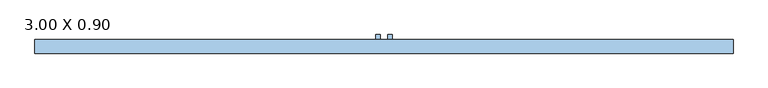
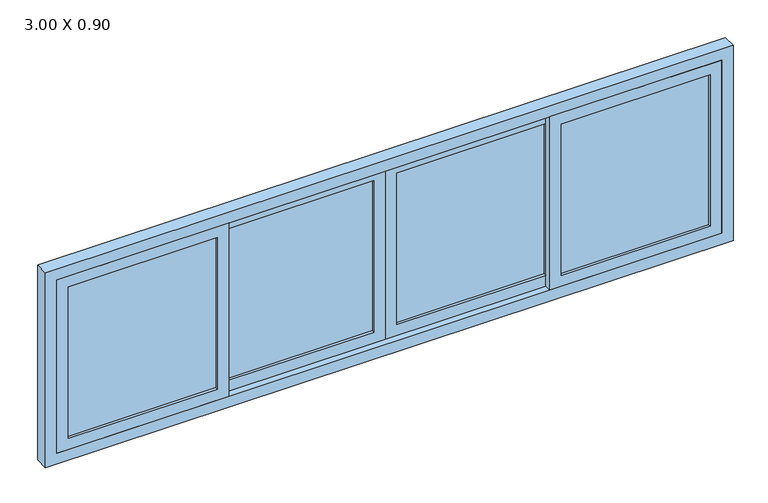
"""IFC4 building model written with IfcOpenShell, lengths in millimetres: window geometry, .CC_ND 300_JANELA_4 FOLHAS DE CORRER_VIDRO : 3.00 X 0.90."""

import ifcopenshell
import ifcopenshell.guid

model = None  # the IFC model being written
_history = None  # IfcOwnerHistory: only IFC2X3 demands one
_inside = {}  # id of a spatial element -> (the spatial element, [elements in it])
_under = {}  # id of a project, library or spatial element -> (it, [spatial elements below it])
_declared = {}  # id of a project -> (the project, [libraries it declares])
_typed = {}  # id of a type object -> (the type object, [elements of that type])
_made_of = {}  # id of a material, layer set ... -> (it, [elements and type objects made of it])


def new_model(schema):
    """Start an empty IFC model of exactly this schema.

    Asked for "IFC4X3", IfcOpenShell would pick the latest addendum, in which some entities
    have other attributes; the version numbers below select the first issue.
    IFC2X3 requires an IfcOwnerHistory on every rooted entity: one is made here for all.
    """
    global model, _history
    if schema == "IFC4X3":
        model = ifcopenshell.file(schema_version=(4, 3, 0, 0))
    else:
        model = ifcopenshell.file(schema=schema)
    _inside.clear()
    _under.clear()
    _declared.clear()
    _typed.clear()
    _made_of.clear()
    _history = None
    if model.schema == "IFC2X3":
        org = make("IfcOrganization", Name="unknown")
        user = make(
            "IfcPersonAndOrganization",
            ThePerson=make("IfcPerson", FamilyName="unknown"),
            TheOrganization=org,
        )
        app = make(
            "IfcApplication",
            ApplicationDeveloper=org,
            Version="unknown",
            ApplicationFullName="unknown",
            ApplicationIdentifier="unknown",
        )
        _history = make(
            "IfcOwnerHistory",
            OwningUser=user,
            OwningApplication=app,
            ChangeAction="ADDED",
            CreationDate=0,
        )
    return model


def make(cls, **values):
    """One entity of the class cls with the attributes given. An attribute that is None is left unset."""
    return model.create_entity(
        cls, **{name: value for name, value in values.items() if value is not None}
    )


def rooted(cls, **values):
    """An entity with a GlobalId (a new one), such as an element, a storey or a relation."""
    return make(cls, GlobalId=ifcopenshell.guid.new(), OwnerHistory=_history, **values)


def si_unit(unit_type, name, prefix=None):
    """IfcSIUnit, for example si_unit("LENGTHUNIT", "METRE", prefix="MILLI")."""
    return make("IfcSIUnit", UnitType=unit_type, Prefix=prefix, Name=name)


def assignment(units):
    """IfcUnitAssignment: the units of a project."""
    return None if units is None else make("IfcUnitAssignment", Units=units)


def point(xyz):
    """IfcCartesianPoint."""
    return None if xyz is None else make("IfcCartesianPoint", Coordinates=xyz)


def direction(xyz):
    """IfcDirection."""
    return None if xyz is None else make("IfcDirection", DirectionRatios=xyz)


def frame(location, z_axis=None, x_axis=None):
    """IfcAxis2Placement3D, a coordinate frame: its origin and axes. An axis left out is left unset."""
    return make(
        "IfcAxis2Placement3D",
        Location=point(location),
        Axis=direction(z_axis),
        RefDirection=direction(x_axis),
    )


def origin():
    """The frame at (0, 0, 0) with its axes left unset."""
    return frame((0.0, 0.0, 0.0))


def place(relative_to, where):
    """IfcLocalPlacement: puts the frame where relative to a parent placement (None: the world)."""
    return make(
        "IfcLocalPlacement", PlacementRelTo=relative_to, RelativePlacement=where
    )


def context(
    kind, dimensions, precision=None, world=None, true_north=None, identifier=None
):
    """IfcGeometricRepresentationContext, for example the 3D "Model" context."""
    return make(
        "IfcGeometricRepresentationContext",
        ContextIdentifier=identifier,
        ContextType=kind,
        CoordinateSpaceDimension=dimensions,
        Precision=precision,
        WorldCoordinateSystem=world,
        TrueNorth=true_north,
    )


def project(units=None, contexts=None):
    """IfcProject with its units and contexts."""
    return rooted(
        "IfcProject",
        Name="project",
        RepresentationContexts=contexts,
        UnitsInContext=assignment(units),
    )


def spatial(cls, under=None, at=None, **own):
    """A site, building, storey or space (cls), placed at a placement, below another one or the project."""
    s = rooted(cls, ObjectPlacement=at, **own)
    if under is not None:
        _under.setdefault(under.id(), (under, []))[1].append(s)
    return s


def polyline(points):
    """IfcPolyline through the points."""
    return make("IfcPolyline", Points=[point(p) for p in points])


def outline(outer, holes=None, kind="AREA"):
    """IfcArbitraryClosedProfileDef: a profile drawn as a closed curve; with holes, ...WithVoids."""
    if holes is None:
        return make("IfcArbitraryClosedProfileDef", ProfileType=kind, OuterCurve=outer)
    return make(
        "IfcArbitraryProfileDefWithVoids",
        ProfileType=kind,
        OuterCurve=outer,
        InnerCurves=holes,
    )


def extrude(swept, where, along, depth):
    """IfcExtrudedAreaSolid: the profile swept, set in the frame where, extruded along a direction by depth."""
    return make(
        "IfcExtrudedAreaSolid",
        SweptArea=swept,
        Position=where,
        ExtrudedDirection=direction(along),
        Depth=depth,
    )


def shape(context_of_items, identifier, shape_type, items):
    """IfcShapeRepresentation: the items that make up one representation, for example the "Body"."""
    return make(
        "IfcShapeRepresentation",
        ContextOfItems=context_of_items,
        RepresentationIdentifier=identifier,
        RepresentationType=shape_type,
        Items=items,
    )


def source(mapping_origin, context_of_items, identifier, shape_type, items):
    """IfcRepresentationMap: a shape defined once, which mapped items show again and again."""
    return make(
        "IfcRepresentationMap",
        MappingOrigin=mapping_origin,
        MappedRepresentation=shape(context_of_items, identifier, shape_type, items),
    )


def transform(
    local_origin,
    x_axis=None,
    y_axis=None,
    z_axis=None,
    scale=None,
    scale2=None,
    scale3=None,
    uniform=True,
):
    """IfcCartesianTransformationOperator3D, or its non-uniform kind. x_axis, y_axis, z_axis: its Axis1, 2, 3."""
    if uniform:
        return make(
            "IfcCartesianTransformationOperator3D",
            Axis1=direction(x_axis),
            Axis2=direction(y_axis),
            LocalOrigin=point(local_origin),
            Scale=scale,
            Axis3=direction(z_axis),
        )
    return make(
        "IfcCartesianTransformationOperator3DnonUniform",
        Axis1=direction(x_axis),
        Axis2=direction(y_axis),
        LocalOrigin=point(local_origin),
        Scale=scale,
        Axis3=direction(z_axis),
        Scale2=scale2,
        Scale3=scale3,
    )


def mapped(mapping_source, mapping_target):
    """IfcMappedItem: shows the shape of a source again, moved by a transform."""
    return make(
        "IfcMappedItem", MappingSource=mapping_source, MappingTarget=mapping_target
    )


def made_of(thing, what):
    """Note that an element or type object is made of a material, layer set ...; save() writes the relation."""
    if what is not None:
        _made_of.setdefault(what.id(), (what, []))[1].append(thing)
    return thing


def element(
    cls,
    number,
    at=None,
    inside=None,
    cuts=None,
    type_object=None,
    material=None,
    context=None,
    identifier="Body",
    shape_type=None,
    held_by="IfcProductDefinitionShape",
    body=None,
    shapes=None,
    **own,
):
    """One element of the class cls, such as IfcWall. Its Tag is "e" and its number.

    at: its placement. inside: the storey or other place that contains it. cuts: it is an
    opening in that element (IfcRelVoidsElement). A single representation is given by context,
    identifier, shape_type and body (its items); several are given by shapes. held_by: the class
    of the entity that holds the representations. save() writes the other relations.
    """
    e = rooted(cls, Tag="e%d" % number, ObjectPlacement=at, **own)
    if body is not None:
        shapes = [shape(context, identifier, shape_type, body)]
    if shapes is not None:
        e.Representation = make(held_by, Representations=shapes)
    if inside is not None:
        _inside.setdefault(inside.id(), (inside, []))[1].append(e)
    if cuts is not None:
        rooted(
            "IfcRelVoidsElement", RelatingBuildingElement=cuts, RelatedOpeningElement=e
        )
    if type_object is not None:
        _typed.setdefault(type_object.id(), (type_object, []))[1].append(e)
    return made_of(e, material)


def aggregate(whole, parts):
    """IfcRelAggregates: a whole, such as a stair, and the parts it consists of."""
    return rooted("IfcRelAggregates", RelatingObject=whole, RelatedObjects=parts)


def save(model, path):
    """Write the relations noted so far, then the file.

    IfcRelAggregates (storeys below a building ...), IfcRelContainedInSpatialStructure (elements
    in a storey), IfcRelDefinesByType, IfcRelAssociatesMaterial and IfcRelDeclares: one each for
    every whole, place, type object, material and project.
    """
    for whole, parts in _under.values():
        aggregate(whole, parts)
    for where, things in _inside.values():
        rooted(
            "IfcRelContainedInSpatialStructure",
            RelatedElements=things,
            RelatingStructure=where,
        )
    for kind, things in _typed.values():
        rooted("IfcRelDefinesByType", RelatedObjects=things, RelatingType=kind)
    for what, things in _made_of.values():
        rooted("IfcRelAssociatesMaterial", RelatedObjects=things, RelatingMaterial=what)
    for by, libraries in _declared.values():
        rooted("IfcRelDeclares", RelatingContext=by, RelatedDefinitions=libraries)
    model.write(path)


def window_3_00_x_0_90_5327f378(model_context):
    return source(origin(), model_context, "Body", "SweptSolid", [
        extrude(outline(polyline([(-50.0, 12.5), (-700.0, 12.5), (-700.0, 17.5), (-50.0, 17.5), (-50.0, 12.5)])), frame((0.0, 0.0, 1100.0), z_axis=(0.0, 0.0, 1.0), x_axis=(1.0, 0.0, 0.0)), (0.0, 0.0, 1.0), 700.0),
        extrude(outline(polyline([(1850.0, 0.0), (1850.0, -750.0), (1050.0, -750.0), (1050.0, 0.0), (1850.0, 0.0)]), holes=[polyline([(1800.0, -50.0), (1100.0, -50.0), (1100.0, -700.0), (1800.0, -700.0), (1800.0, -50.0)])]), frame((0.0, 0.0, 0.0), z_axis=(0.0, 1.0, 0.0), x_axis=(0.0, 0.0, 1.0)), (0.0, 0.0, 1.0), 30.0),
        extrude(outline(polyline([(-750.0, -17.5), (-1400.0, -17.5), (-1400.0, -12.5), (-750.0, -12.5), (-750.0, -17.5)])), frame((0.0, 0.0, 1100.0), z_axis=(0.0, 0.0, 1.0), x_axis=(1.0, 0.0, 0.0)), (0.0, 0.0, 1.0), 700.0),
        extrude(outline(polyline([(1850.0, -700.0), (1850.0, -1450.0), (1050.0, -1450.0), (1050.0, -700.0), (1850.0, -700.0)]), holes=[polyline([(1800.0, -750.0), (1100.0, -750.0), (1100.0, -1400.0), (1800.0, -1400.0), (1800.0, -750.0)])]), frame((0.0, -30.0, 0.0), z_axis=(0.0, 1.0, 0.0), x_axis=(0.0, 0.0, 1.0)), (0.0, 0.0, 1.0), 30.0),
        extrude(outline(polyline([(1400.0, -17.5), (750.0, -17.5), (750.0, -12.5), (1400.0, -12.5), (1400.0, -17.5)])), frame((0.0, 0.0, 1100.0), z_axis=(0.0, 0.0, 1.0), x_axis=(1.0, 0.0, 0.0)), (0.0, 0.0, 1.0), 700.0),
        extrude(outline(polyline([(1850.0, 1450.0), (1850.0, 700.0), (1050.0, 700.0), (1050.0, 1450.0), (1850.0, 1450.0)]), holes=[polyline([(1800.0, 1400.0), (1100.0, 1400.0), (1100.0, 750.0), (1800.0, 750.0), (1800.0, 1400.0)])]), frame((0.0, -30.0, 0.0), z_axis=(0.0, 1.0, 0.0), x_axis=(0.0, 0.0, 1.0)), (0.0, 0.0, 1.0), 30.0),
        extrude(outline(polyline([(700.0, 12.5), (50.0, 12.5), (50.0, 17.5), (700.0, 17.5), (700.0, 12.5)])), frame((0.0, 0.0, 1100.0), z_axis=(0.0, 0.0, 1.0), x_axis=(1.0, 0.0, 0.0)), (0.0, 0.0, 1.0), 700.0),
        extrude(outline(polyline([(1850.0, 750.0), (1850.0, 0.0), (1050.0, 0.0), (1050.0, 750.0), (1850.0, 750.0)]), holes=[polyline([(1800.0, 700.0), (1100.0, 700.0), (1100.0, 50.0), (1800.0, 50.0), (1800.0, 700.0)])]), frame((0.0, 0.0, 0.0), z_axis=(0.0, 1.0, 0.0), x_axis=(0.0, 0.0, 1.0)), (0.0, 0.0, 1.0), 30.0),
        extrude(outline(polyline([(1900.0, -1500.0), (1000.0, -1500.0), (1000.0, 1500.0), (1900.0, 1500.0), (1900.0, -1500.0)]), holes=[polyline([(1050.0, -1450.0), (1850.0, -1450.0), (1850.0, 1450.0), (1050.0, 1450.0), (1050.0, -1450.0)])]), frame((0.0, -30.0, 0.0), z_axis=(0.0, 1.0, 0.0), x_axis=(0.0, 0.0, 1.0)), (0.0, 0.0, 1.0), 60.0),
        extrude(outline(polyline([(-35.9492003, 30.0), (-35.9492003, 50.0), (-15.9492003, 50.0), (-15.9492003, 30.0), (-35.9492003, 30.0)])), frame((0.0, 0.0, 1390.0), z_axis=(0.0, 0.0, 1.0), x_axis=(1.0, 0.0, 0.0)), (0.0, 0.0, 1.0), 120.0),
        extrude(outline(polyline([(15.9492003, 30.0), (15.9492003, 50.0), (35.9492003, 50.0), (35.9492003, 30.0), (15.9492003, 30.0)])), frame((0.0, 0.0, 1390.0), z_axis=(0.0, 0.0, 1.0), x_axis=(1.0, 0.0, 0.0)), (0.0, 0.0, 1.0), 120.0),
    ])


if __name__ == "__main__":
    model = new_model("IFC4")
    model_context = context("Model", 3, world=origin())
    ifc_project = project(units=[si_unit("LENGTHUNIT", "METRE", prefix="MILLI")], contexts=[model_context])
    site = spatial("IfcSite", under=ifc_project)
    building = spatial("IfcBuilding", under=site)
    placement = place(None, origin())
    window_3_00_x_0_90_shape = window_3_00_x_0_90_5327f378(model_context)
    element("IfcWindow", 1, ObjectType=".CC_ND 300_JANELA_4 FOLHAS DE CORRER_VIDRO : 3.00 X 0.90", at=placement, inside=building, context=model_context, shape_type="MappedRepresentation", body=[
        mapped(window_3_00_x_0_90_shape, transform((0.0, 0.0, 0.0), x_axis=(1.0, 0.0, 0.0), y_axis=(0.0, 1.0, 0.0), z_axis=(0.0, 0.0, 1.0))),
    ])
    save(model, "model.ifc")

# Revit data of these elements
# Type ".CC_ND 300_JANELA_4 FOLHAS DE CORRER_VIDRO : 3.00 X 0.90"
#   Type Mark = "61"
#   Largura moldura = 0.06 m
#   Largura janela = 2.90 m
#   Largura esquadria = 0.05 m
#   Largura do painel = 0.75 m
#   Largura da moldura do painel = 0.05 m
#   Espessura painel = 0.03 m
#   Espessura moldura = 0.03 m
#   Altura janela = 0.80 m
#   Height = 0.90 m
#   Altura-padrão do peitoril = 1.00 m
#   Width = 3.00 m
#   Puxadores [instance default] = yes
#   Moldura interna [instance default] = yes
#   Moldura externa [instance default] = yes
#   Tipo de vidro = .VIDRO GENÉRICO
#   Material puxadores = .ALUMÍNIO COM PINTURA ELETROSTÁTICA BRANCA
#   Material moldura = .ALUMÍNIO COM PINTURA ELETROSTÁTICA BRANCA
#   Material da esquadria = .ALUMÍNIO COM PINTURA ELETROSTÁTICA BRANCA
#   Wall Closure = (empty or 0)
# Element 1 (IfcWindow, ".CC_ND 300_JANELA_4 FOLHAS DE CORRER_VIDRO : 3.00 X 0.90")
#   Moldura interna = no
#   Moldura externa = no
#   Materials on its faces: ".ALUMÍNIO COM PINTURA ELETROSTÁTICA BRANCA", ".VIDRO GENÉRICO"
# Materials
#   ".VIDRO GENÉRICO": class ".CC_VIDRO", colour RGB 0 128 192, transparency 0.9, Description = "Vidro comum", Cost = 0
#   ".ALUMÍNIO COM PINTURA ELETROSTÁTICA BRANCA": class "CC_METAIS", colour RGB 241 241 241, transparency 0, Cost = 0
